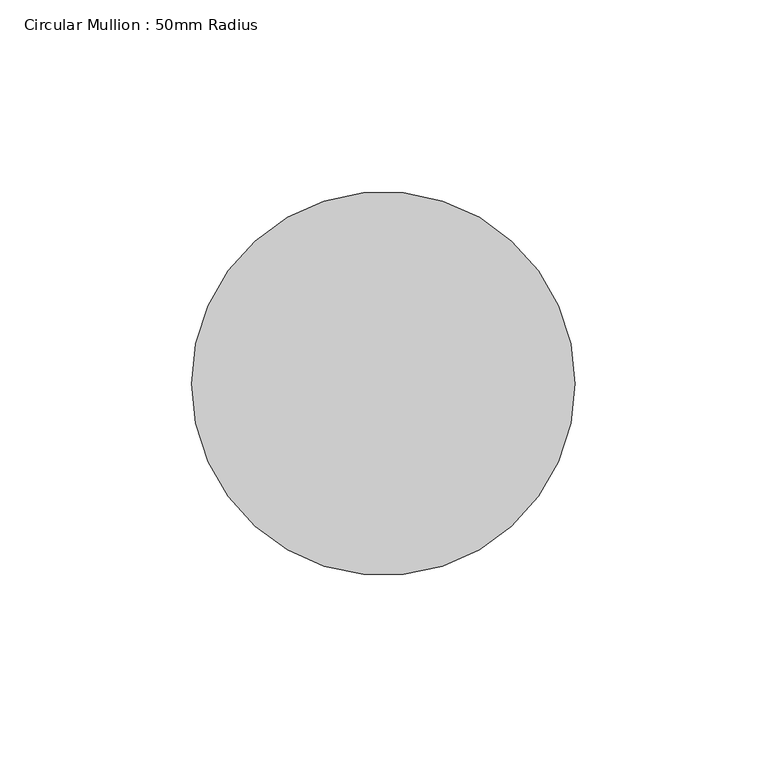
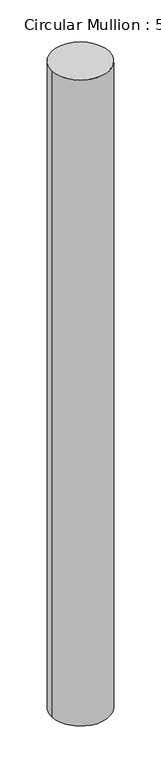
"""IFC4 building model written with IfcOpenShell, lengths in millimetres: member geometry, Circular Mullion : 50mm Radius."""

from ifc_helpers import new_model, si_unit, point, frame, origin, origin_2d, place, context, project, spatial, circle_curve, trimmed, segment, composite_curve, outline, extrude, source, transform, mapped, element, save


def circular_mullion_50mm_radius_40b2a3be(model_context):
    return source(origin(), model_context, "Body", "SweptSolid", [
        extrude(outline(composite_curve([segment(trimmed(circle_curve(origin_2d(), 50.0), [point((50.0, 0.0))], [point((-50.0, 0.0))], False, "CARTESIAN"), True, "CONTINUOUS"), segment(trimmed(circle_curve(origin_2d(), 50.0), [point((-50.0, 0.0))], [point((50.0, 0.0))], False, "CARTESIAN"), True, "CONTINUOUS")], self_intersect=False)), frame((0.0, 0.0, -1184.4580735), z_axis=(0.0, 0.0, 1.0), x_axis=(1.0, 0.0, 0.0)), (0.0, 0.0, 1.0), 1184.4580735),
    ])


if __name__ == "__main__":
    model = new_model("IFC4")
    model_context = context("Model", 3, world=origin())
    ifc_project = project(units=[si_unit("LENGTHUNIT", "METRE", prefix="MILLI")], contexts=[model_context])
    site = spatial("IfcSite", under=ifc_project)
    building = spatial("IfcBuilding", under=site)
    placement = place(None, origin())
    circular_mullion_50mm_radius_shape = circular_mullion_50mm_radius_40b2a3be(model_context)
    element("IfcMember", 1, ObjectType="Circular Mullion : 50mm Radius", at=placement, inside=building, context=model_context, shape_type="MappedRepresentation", body=[
        mapped(circular_mullion_50mm_radius_shape, transform((0.0, 0.0, 0.0), x_axis=(1.0, 0.0, 0.0), y_axis=(0.0, 1.0, 0.0), z_axis=(0.0, 0.0, 1.0))),
    ])
    save(model, "model.ifc")

# Revit data of these elements
# Type "Circular Mullion : 50mm Radius"
#   built-in parameter 1007350 = 0.164042 (stored number, unit not read)
# Element 1 (IfcMember, "Circular Mullion : 50mm Radius")
#   Materials on its faces: "Aluminium"
# Materials
#   "Aluminium": class "Metal", colour RGB 247 247 247, transparency 0, Description = "Aluminium 6061", Cost = 0
